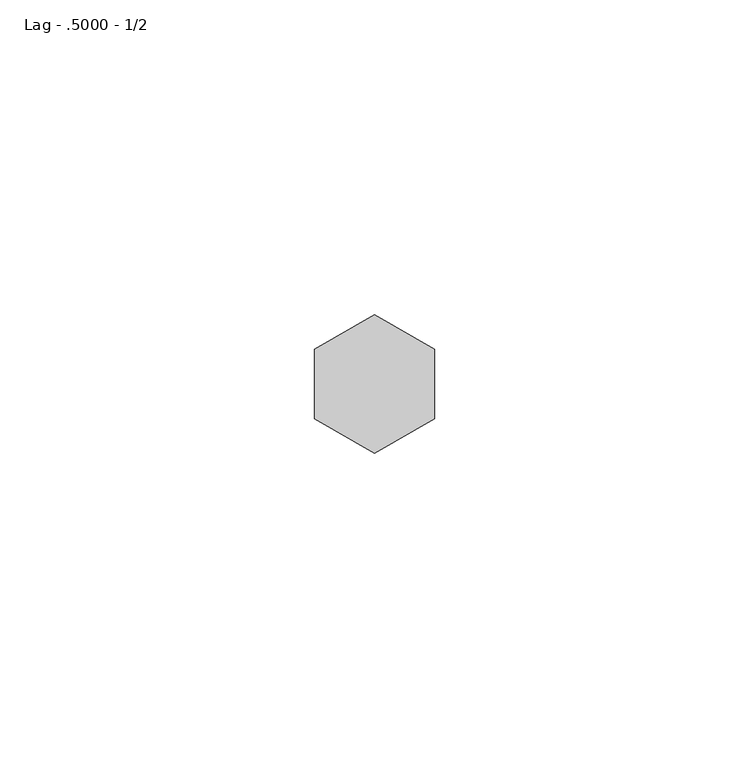
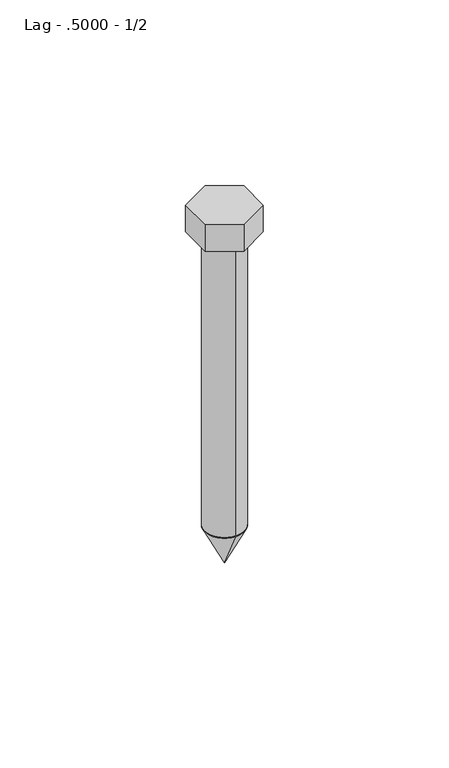
"""IFC4 building model written with IfcOpenShell, lengths in millimetres: fastener geometry, 060523 - W_P_C - Fastenings - Generic : Lag - .5000 - 1/2."""

from ifc_helpers import new_model, si_unit, point, frame, origin, origin_with_axes, origin_2d, place, context, project, spatial, polyline, circle_curve, trimmed, segment, composite_curve, outline, extrude, source, transform, mapped, element, save
from ifc_brep_helpers import plane_surface, revolved_surface, advanced_brep


def lag_5000_1_2_a2b3b2fc(model_context):
    return source(origin(), model_context, "Body", "SolidModel", [
        advanced_brep(
        [(0.0, -6.5484375, -101.6), (0.0, 6.5484375, -101.6), (0.0, 0.0, -101.6), (0.0, 0.0, -114.696875)],
        [
            (0, 1, circle_curve(frame((0.0, 0.0, -101.6), z_axis=(0.0, 0.0, 1.0), x_axis=(0.0, 1.0, 0.0)), 6.5484375)),
            (1, 2),
            (2, 0),
            (1, 0, circle_curve(frame((0.0, 0.0, -101.6), z_axis=(0.0, 0.0, 1.0), x_axis=(0.0, 1.0, 0.0)), 6.5484375)),
            (3, 1),
            (0, 3),
        ],
        [
            plane_surface(frame((0.0, 0.0, -101.6), z_axis=(0.0, 0.0, 1.0), x_axis=(0.0, 1.0, 0.0))),
            revolved_surface(polyline([(0.0, 6.5484375, -101.6), (0.0, 0.0, -114.696875)]), (0.0, 0.0, -103.0840259), (0.0, 0.0, -1.0)),
        ],
        [
            (0, [[1, 2, 3]]),
            (0, [[4, -3, -2]]),
            (1, [[5, -1, 6]]),
            (1, [[-6, -4, -5]]),
        ],
    ),
        extrude(outline(polyline([(-9.525, 5.4992613), (0.0, 10.9985226), (9.525, 5.4992613), (9.525, -5.4992613), (0.0, -10.9985226), (-9.525, -5.4992613), (-9.525, 5.4992613)])), origin_with_axes(), (0.0, 0.0, 1.0), 9.2273437),
        extrude(outline(composite_curve([segment(trimmed(circle_curve(origin_2d(), 6.5484375), [point((0.0, -6.5484375))], [point((0.0, 6.5484375))], False, "CARTESIAN"), True, "CONTINUOUS"), segment(trimmed(circle_curve(origin_2d(), 6.5484375), [point((0.0, 6.5484375))], [point((0.0, -6.5484375))], False, "CARTESIAN"), True, "CONTINUOUS")], self_intersect=False)), frame((0.0, 0.0, -101.6), z_axis=(0.0, 0.0, 1.0), x_axis=(1.0, 0.0, 0.0)), (0.0, 0.0, 1.0), 101.6),
    ])


if __name__ == "__main__":
    model = new_model("IFC4")
    model_context = context("Model", 3, world=origin())
    ifc_project = project(units=[si_unit("LENGTHUNIT", "METRE", prefix="MILLI")], contexts=[model_context])
    site = spatial("IfcSite", under=ifc_project)
    building = spatial("IfcBuilding", under=site)
    placement = place(None, origin())
    lag_5000_1_2_shape = lag_5000_1_2_a2b3b2fc(model_context)
    element("IfcFastener", 1, ObjectType="060523 - W_P_C - Fastenings - Generic : Lag - .5000 - 1/2", at=placement, inside=building, context=model_context, shape_type="MappedRepresentation", body=[
        mapped(lag_5000_1_2_shape, transform((0.0, 0.0, 0.0), x_axis=(1.0, 0.0, 0.0), y_axis=(0.0, 1.0, 0.0), z_axis=(0.0, 0.0, 1.0))),
    ])
    save(model, "model.ifc")

# Revit data of these elements
# Type "060523 - W_P_C - Fastenings - Generic : Lag - .5000 - 1/2"
#   Washer_Thickness = 0' - 0 31/256"
#   Washer Radius = 0' - 0 159/256"
#   Washer Offset - Head = 0' - 0"
#   Washer Offset = 0' - 0"
#   Thickness_of_Substrate [instance default] = 0' - 1"
#   Side = 0' - 0 111/256"
#   Radius = 0' - 0 33/128"
#   Length [instance default] = 0' - 4"
#   Head Size = 0' - 0 3/4"
#   Head Radius = 0' - 0 3/8"
#   Head Height = 0' - 0 93/256"
#   Double Diameter = 0' - 1 1/32"
#   Diameter = 0' - 0 33/64"
#   Default Elevation = 4' - 0"
#   Washer_Nut_Visibility = no
#   Washer_Head_Visibility = no
#   Round_Head_Visibility = no
#   Point Visibility = yes
#   Nut_Visibility = no
#   Hex_Head_Visiblilty = yes
#   Washer Material = none
#   Bolt Material (Size) = AT SILL - FASTENER AT 24" O.C.
# Element 1 (IfcFastener, "060523 - W_P_C - Fastenings - Generic : Lag - .5000 - 1/2")
#   Materials on its faces: "AT SILL - FASTENER AT 24\" O.C."
# Materials
#   "AT SILL - FASTENER AT 24\" O.C.": class "Generic", colour RGB 120 120 120, transparency 0, Cost = 0
